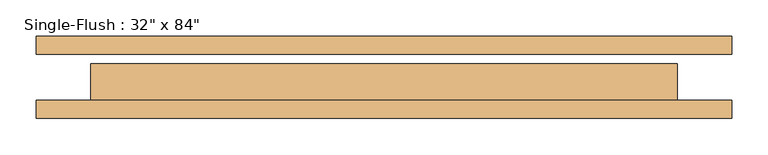
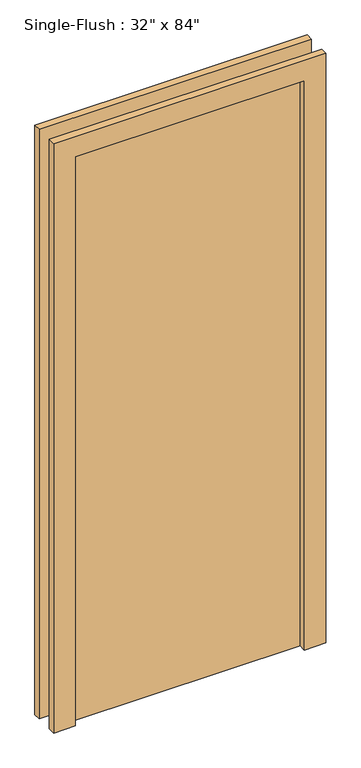
"""IFC4 building model written with IfcOpenShell, lengths in millimetres: door geometry."""

from ifc_helpers import new_model, si_unit, frame, origin, origin_with_axes, place, context, project, spatial, polyline, outline, extrude, source, transform, mapped, element, save


def door_9a041354(model_context):
    return source(origin(), model_context, "Body", "SweptSolid", [
        extrude(outline(polyline([(2209.8, -482.6), (0.0, -482.6), (0.0, -406.4), (2133.6, -406.4), (2133.6, 406.4), (0.0, 406.4), (0.0, 482.6), (2209.8, 482.6), (2209.8, -482.6)])), frame((0.0, -57.15, 0.0), z_axis=(0.0, 1.0, 0.0), x_axis=(0.0, 0.0, 1.0)), (0.0, 0.0, 1.0), 25.4),
        extrude(outline(polyline([(2209.8, 482.6), (2209.8, -482.6), (0.0, -482.6), (0.0, -406.4), (2133.6, -406.4), (2133.6, 406.4), (0.0, 406.4), (0.0, 482.6), (2209.8, 482.6)])), frame((0.0, 31.75, 0.0), z_axis=(0.0, 1.0, 0.0), x_axis=(0.0, 0.0, 1.0)), (0.0, 0.0, 1.0), 25.4),
        extrude(outline(polyline([(406.4, 19.05), (406.4, -31.75), (-406.4, -31.75), (-406.4, 19.05), (406.4, 19.05)])), origin_with_axes(), (0.0, 0.0, 1.0), 2133.6),
    ])


if __name__ == "__main__":
    model = new_model("IFC4")
    model_context = context("Model", 3, world=origin())
    ifc_project = project(units=[si_unit("LENGTHUNIT", "METRE", prefix="MILLI")], contexts=[model_context])
    site = spatial("IfcSite", under=ifc_project)
    building = spatial("IfcBuilding", under=site)
    placement = place(None, origin())
    door_shape = door_9a041354(model_context)
    element("IfcDoor", 1, ObjectType="Single-Flush : 32\" x 84\"", at=placement, inside=building, context=model_context, shape_type="MappedRepresentation", body=[
        mapped(door_shape, transform((0.0, 0.0, 0.0), x_axis=(1.0, 0.0, 0.0), y_axis=(0.0, 1.0, 0.0), z_axis=(0.0, 0.0, 1.0))),
    ])
    save(model, "model.ifc")

# Revit data of these elements
# Type "Single-Flush : 32\" x 84\""
#   Type Mark = "3"
#   Construction Type Id = "MDOOR"
#   Assembly Code = "C1020"
#   Analytic Construction = "Metal"
#   Thickness = 0' - 2"
#   Heat Transfer Coefficient (U) = 0.651978 BTU/(h·ft²·°F)
#   Height = 7' - 0"
#   Trim Projection Ext = 0' - 1"
#   Trim Projection Int = 0' - 1"
#   Trim Width = 0' - 3"
#   Width = 2' - 8"
#   Define Thermal Properties by = 1
#   Define Thermal Properties by = 1
#   Door Material = Door - Panel
#   Frame Material = Door - Frame
#   Visual Light Transmittance = 0
#   Solar Heat Gain Coefficient = 0
#   Function = (empty or 0)
#   Wall Closure = (empty or 0)
# Element 1 (IfcDoor, "Single-Flush : 32\" x 84\"")
#   Materials on its faces: "Door - Frame", "Door - Panel"
# Materials
#   "Door - Panel": class "Wood", colour RGB 210 159 95, transparency 0, Cost = 0
#   "Door - Frame": class "Miscellaneous", colour RGB 118 70 51, transparency 0, Cost = 0
